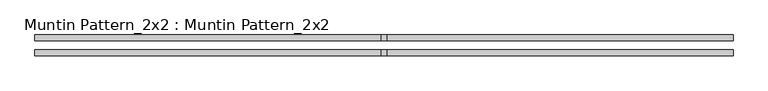
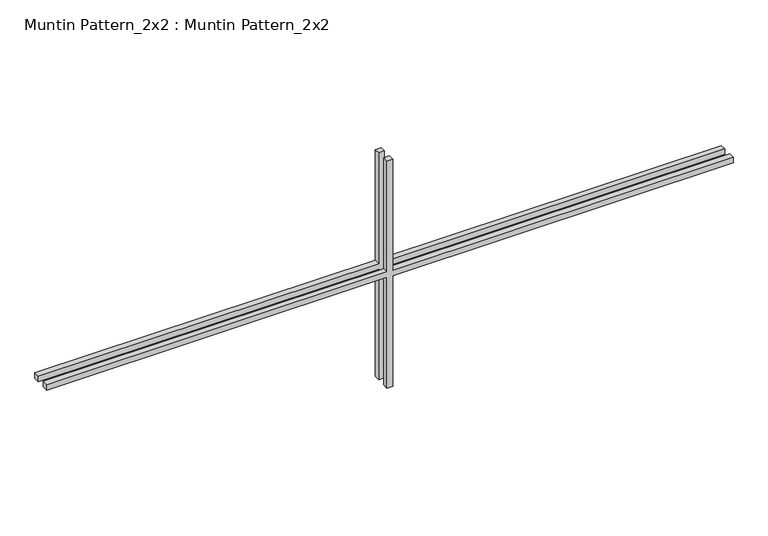
"""IFC4 building model written with IfcOpenShell, lengths in millimetres: proxy geometry, Muntin Pattern_2x2 : Muntin Pattern_2x2."""

import ifcopenshell
import ifcopenshell.guid

model = None  # the IFC model being written
_history = None  # IfcOwnerHistory: only IFC2X3 demands one
_inside = {}  # id of a spatial element -> (the spatial element, [elements in it])
_under = {}  # id of a project, library or spatial element -> (it, [spatial elements below it])
_declared = {}  # id of a project -> (the project, [libraries it declares])
_typed = {}  # id of a type object -> (the type object, [elements of that type])
_made_of = {}  # id of a material, layer set ... -> (it, [elements and type objects made of it])


def new_model(schema):
    """Start an empty IFC model of exactly this schema.

    Asked for "IFC4X3", IfcOpenShell would pick the latest addendum, in which some entities
    have other attributes; the version numbers below select the first issue.
    IFC2X3 requires an IfcOwnerHistory on every rooted entity: one is made here for all.
    """
    global model, _history
    if schema == "IFC4X3":
        model = ifcopenshell.file(schema_version=(4, 3, 0, 0))
    else:
        model = ifcopenshell.file(schema=schema)
    _inside.clear()
    _under.clear()
    _declared.clear()
    _typed.clear()
    _made_of.clear()
    _history = None
    if model.schema == "IFC2X3":
        org = make("IfcOrganization", Name="unknown")
        user = make(
            "IfcPersonAndOrganization",
            ThePerson=make("IfcPerson", FamilyName="unknown"),
            TheOrganization=org,
        )
        app = make(
            "IfcApplication",
            ApplicationDeveloper=org,
            Version="unknown",
            ApplicationFullName="unknown",
            ApplicationIdentifier="unknown",
        )
        _history = make(
            "IfcOwnerHistory",
            OwningUser=user,
            OwningApplication=app,
            ChangeAction="ADDED",
            CreationDate=0,
        )
    return model


def make(cls, **values):
    """One entity of the class cls with the attributes given. An attribute that is None is left unset."""
    return model.create_entity(
        cls, **{name: value for name, value in values.items() if value is not None}
    )


def rooted(cls, **values):
    """An entity with a GlobalId (a new one), such as an element, a storey or a relation."""
    return make(cls, GlobalId=ifcopenshell.guid.new(), OwnerHistory=_history, **values)


def si_unit(unit_type, name, prefix=None):
    """IfcSIUnit, for example si_unit("LENGTHUNIT", "METRE", prefix="MILLI")."""
    return make("IfcSIUnit", UnitType=unit_type, Prefix=prefix, Name=name)


def assignment(units):
    """IfcUnitAssignment: the units of a project."""
    return None if units is None else make("IfcUnitAssignment", Units=units)


def point(xyz):
    """IfcCartesianPoint."""
    return None if xyz is None else make("IfcCartesianPoint", Coordinates=xyz)


def direction(xyz):
    """IfcDirection."""
    return None if xyz is None else make("IfcDirection", DirectionRatios=xyz)


def frame(location, z_axis=None, x_axis=None):
    """IfcAxis2Placement3D, a coordinate frame: its origin and axes. An axis left out is left unset."""
    return make(
        "IfcAxis2Placement3D",
        Location=point(location),
        Axis=direction(z_axis),
        RefDirection=direction(x_axis),
    )


def origin():
    """The frame at (0, 0, 0) with its axes left unset."""
    return frame((0.0, 0.0, 0.0))


def place(relative_to, where):
    """IfcLocalPlacement: puts the frame where relative to a parent placement (None: the world)."""
    return make(
        "IfcLocalPlacement", PlacementRelTo=relative_to, RelativePlacement=where
    )


def context(
    kind, dimensions, precision=None, world=None, true_north=None, identifier=None
):
    """IfcGeometricRepresentationContext, for example the 3D "Model" context."""
    return make(
        "IfcGeometricRepresentationContext",
        ContextIdentifier=identifier,
        ContextType=kind,
        CoordinateSpaceDimension=dimensions,
        Precision=precision,
        WorldCoordinateSystem=world,
        TrueNorth=true_north,
    )


def project(units=None, contexts=None):
    """IfcProject with its units and contexts."""
    return rooted(
        "IfcProject",
        Name="project",
        RepresentationContexts=contexts,
        UnitsInContext=assignment(units),
    )


def spatial(cls, under=None, at=None, **own):
    """A site, building, storey or space (cls), placed at a placement, below another one or the project."""
    s = rooted(cls, ObjectPlacement=at, **own)
    if under is not None:
        _under.setdefault(under.id(), (under, []))[1].append(s)
    return s


def polyline(points):
    """IfcPolyline through the points."""
    return make("IfcPolyline", Points=[point(p) for p in points])


def outline(outer, holes=None, kind="AREA"):
    """IfcArbitraryClosedProfileDef: a profile drawn as a closed curve; with holes, ...WithVoids."""
    if holes is None:
        return make("IfcArbitraryClosedProfileDef", ProfileType=kind, OuterCurve=outer)
    return make(
        "IfcArbitraryProfileDefWithVoids",
        ProfileType=kind,
        OuterCurve=outer,
        InnerCurves=holes,
    )


def extrude(swept, where, along, depth):
    """IfcExtrudedAreaSolid: the profile swept, set in the frame where, extruded along a direction by depth."""
    return make(
        "IfcExtrudedAreaSolid",
        SweptArea=swept,
        Position=where,
        ExtrudedDirection=direction(along),
        Depth=depth,
    )


def shape(context_of_items, identifier, shape_type, items):
    """IfcShapeRepresentation: the items that make up one representation, for example the "Body"."""
    return make(
        "IfcShapeRepresentation",
        ContextOfItems=context_of_items,
        RepresentationIdentifier=identifier,
        RepresentationType=shape_type,
        Items=items,
    )


def source(mapping_origin, context_of_items, identifier, shape_type, items):
    """IfcRepresentationMap: a shape defined once, which mapped items show again and again."""
    return make(
        "IfcRepresentationMap",
        MappingOrigin=mapping_origin,
        MappedRepresentation=shape(context_of_items, identifier, shape_type, items),
    )


def transform(
    local_origin,
    x_axis=None,
    y_axis=None,
    z_axis=None,
    scale=None,
    scale2=None,
    scale3=None,
    uniform=True,
):
    """IfcCartesianTransformationOperator3D, or its non-uniform kind. x_axis, y_axis, z_axis: its Axis1, 2, 3."""
    if uniform:
        return make(
            "IfcCartesianTransformationOperator3D",
            Axis1=direction(x_axis),
            Axis2=direction(y_axis),
            LocalOrigin=point(local_origin),
            Scale=scale,
            Axis3=direction(z_axis),
        )
    return make(
        "IfcCartesianTransformationOperator3DnonUniform",
        Axis1=direction(x_axis),
        Axis2=direction(y_axis),
        LocalOrigin=point(local_origin),
        Scale=scale,
        Axis3=direction(z_axis),
        Scale2=scale2,
        Scale3=scale3,
    )


def mapped(mapping_source, mapping_target):
    """IfcMappedItem: shows the shape of a source again, moved by a transform."""
    return make(
        "IfcMappedItem", MappingSource=mapping_source, MappingTarget=mapping_target
    )


def made_of(thing, what):
    """Note that an element or type object is made of a material, layer set ...; save() writes the relation."""
    if what is not None:
        _made_of.setdefault(what.id(), (what, []))[1].append(thing)
    return thing


def element(
    cls,
    number,
    at=None,
    inside=None,
    cuts=None,
    type_object=None,
    material=None,
    context=None,
    identifier="Body",
    shape_type=None,
    held_by="IfcProductDefinitionShape",
    body=None,
    shapes=None,
    **own,
):
    """One element of the class cls, such as IfcWall. Its Tag is "e" and its number.

    at: its placement. inside: the storey or other place that contains it. cuts: it is an
    opening in that element (IfcRelVoidsElement). A single representation is given by context,
    identifier, shape_type and body (its items); several are given by shapes. held_by: the class
    of the entity that holds the representations. save() writes the other relations.
    """
    e = rooted(cls, Tag="e%d" % number, ObjectPlacement=at, **own)
    if body is not None:
        shapes = [shape(context, identifier, shape_type, body)]
    if shapes is not None:
        e.Representation = make(held_by, Representations=shapes)
    if inside is not None:
        _inside.setdefault(inside.id(), (inside, []))[1].append(e)
    if cuts is not None:
        rooted(
            "IfcRelVoidsElement", RelatingBuildingElement=cuts, RelatedOpeningElement=e
        )
    if type_object is not None:
        _typed.setdefault(type_object.id(), (type_object, []))[1].append(e)
    return made_of(e, material)


def aggregate(whole, parts):
    """IfcRelAggregates: a whole, such as a stair, and the parts it consists of."""
    return rooted("IfcRelAggregates", RelatingObject=whole, RelatedObjects=parts)


def save(model, path):
    """Write the relations noted so far, then the file.

    IfcRelAggregates (storeys below a building ...), IfcRelContainedInSpatialStructure (elements
    in a storey), IfcRelDefinesByType, IfcRelAssociatesMaterial and IfcRelDeclares: one each for
    every whole, place, type object, material and project.
    """
    for whole, parts in _under.values():
        aggregate(whole, parts)
    for where, things in _inside.values():
        rooted(
            "IfcRelContainedInSpatialStructure",
            RelatedElements=things,
            RelatingStructure=where,
        )
    for kind, things in _typed.values():
        rooted("IfcRelDefinesByType", RelatedObjects=things, RelatingType=kind)
    for what, things in _made_of.values():
        rooted("IfcRelAssociatesMaterial", RelatedObjects=things, RelatingMaterial=what)
    for by, libraries in _declared.values():
        rooted("IfcRelDeclares", RelatingContext=by, RelatedDefinitions=libraries)
    model.write(path)


def muntin_pattern_2x2_muntin_pattern_2x2_54380e04(model_context):
    return source(origin(), model_context, "Body", "SweptSolid", [
        extrude(outline(polyline([(268.2875, -6.35), (268.2875, -749.3), (255.5875, -749.3), (255.5875, -6.35), (0.0, -6.35), (0.0, 6.35), (255.5875, 6.35), (255.5875, 749.3), (268.2875, 749.3), (268.2875, 6.35), (523.875, 6.35), (523.875, -6.35), (268.2875, -6.35)])), frame((0.0, 9.525, 0.0), z_axis=(0.0, 1.0, 0.0), x_axis=(0.0, 0.0, 1.0)), (0.0, 0.0, 1.0), 12.7),
        extrude(outline(polyline([(268.2875, -6.35), (268.2875, -749.3), (255.5875, -749.3), (255.5875, -6.35), (0.0, -6.35), (0.0, 6.35), (255.5875, 6.35), (255.5875, 749.3), (268.2875, 749.3), (268.2875, 6.35), (523.875, 6.35), (523.875, -6.35), (268.2875, -6.35)])), frame((0.0, -22.225, 0.0), z_axis=(0.0, 1.0, 0.0), x_axis=(0.0, 0.0, 1.0)), (0.0, 0.0, 1.0), 12.7),
    ])


if __name__ == "__main__":
    model = new_model("IFC4")
    model_context = context("Model", 3, world=origin())
    ifc_project = project(units=[si_unit("LENGTHUNIT", "METRE", prefix="MILLI")], contexts=[model_context])
    site = spatial("IfcSite", under=ifc_project)
    building = spatial("IfcBuilding", under=site)
    placement = place(None, origin())
    muntin_pattern_2x2_muntin_pattern_2x2_shape = muntin_pattern_2x2_muntin_pattern_2x2_54380e04(model_context)
    element("IfcBuildingElementProxy", 1, Name="Muntin Pattern_2x2 : Muntin Pattern_2x2", ObjectType="Muntin Pattern_2x2 : Muntin Pattern_2x2", at=placement, inside=building, context=model_context, shape_type="MappedRepresentation", body=[
        mapped(muntin_pattern_2x2_muntin_pattern_2x2_shape, transform((0.0, 0.0, 0.0), x_axis=(1.0, 0.0, 0.0), y_axis=(0.0, 1.0, 0.0), z_axis=(0.0, 0.0, 1.0))),
    ])
    save(model, "model.ifc")

# Revit data of these elements
# Type "Muntin Pattern_2x2 : Muntin Pattern_2x2"
#   Width [instance default] = 4' - 0"
#   Thickness = 0' - 0 1/2"
#   Height [instance default] = 4' - 0"
#   Distance = 0' - 0 3/4"
#   Interior Material [instance default] = none
#   Exterior Material [instance default] = none
# Element 1 (IfcBuildingElementProxy, "Muntin Pattern_2x2 : Muntin Pattern_2x2")
#   Width = 4' - 11"
#   Height = 1' - 8 5/8"
#   Interior Material = Wood - Stained
#   Exterior Material = Clad - White
#   Materials on its faces: "Clad - White", "Wood - Stained"
# Materials
#   "Clad - White": class "Wood", colour RGB 242 242 238, transparency 0, Cost = 0
#   "Wood - Stained": class "Wood", colour RGB 224 178 126, transparency 0, Cost = 0
